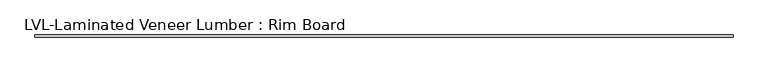
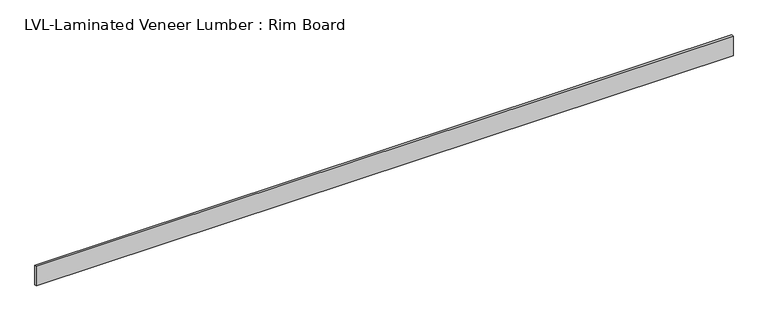
"""IFC4 building model written with IfcOpenShell, lengths in millimetres: beam geometry, LVL-Laminated Veneer Lumber : Rim Board."""

from ifc_helpers import new_model, si_unit, frame, origin, place, context, project, spatial, polyline, outline, extrude, source, transform, mapped, element, save


def lvl_laminated_veneer_lumber_rim_board_c76fbf88(model_context):
    return source(origin(), model_context, "Body", "SweptSolid", [
        extrude(outline(polyline([(5118.89375, 15.875), (5118.89375, -15.875), (-5118.89375, -15.875), (-5118.89375, 15.875), (5118.89375, 15.875)])), frame((0.0, 0.0, -150.8125), z_axis=(0.0, 0.0, 1.0), x_axis=(1.0, 0.0, 0.0)), (0.0, 0.0, 1.0), 301.625),
    ])


if __name__ == "__main__":
    model = new_model("IFC4")
    model_context = context("Model", 3, world=origin())
    ifc_project = project(units=[si_unit("LENGTHUNIT", "METRE", prefix="MILLI")], contexts=[model_context])
    site = spatial("IfcSite", under=ifc_project)
    building = spatial("IfcBuilding", under=site)
    placement = place(None, origin())
    lvl_laminated_veneer_lumber_rim_board_shape = lvl_laminated_veneer_lumber_rim_board_c76fbf88(model_context)
    element("IfcBeam", 1, ObjectType="LVL-Laminated Veneer Lumber : Rim Board", at=placement, inside=building, context=model_context, shape_type="MappedRepresentation", body=[
        mapped(lvl_laminated_veneer_lumber_rim_board_shape, transform((0.0, 0.0, 0.0), x_axis=(1.0, 0.0, 0.0), y_axis=(0.0, 1.0, 0.0), z_axis=(0.0, 0.0, 1.0))),
    ])
    save(model, "model.ifc")

# Revit data of these elements
# Type "LVL-Laminated Veneer Lumber : Rim Board"
#   Assembly Code = "B10"
#   Cost = 4.6
#   Length [instance default] = 5' - 0"
#   b = 0' - 1 1/4"
#   d = 0' - 11 7/8"
#   Structural Material [instance default] = Softwood, Lumber
# Element 1 (IfcBeam, "LVL-Laminated Veneer Lumber : Rim Board")
#   Structural Material = Douglas Fir #2
#   Materials on its faces: "Douglas Fir #2"
# Materials
#   "Softwood, Lumber": class "Wood", colour RGB 223 192 134, transparency 0, Description = "Pinus Echinata", Cost = 0
#   "Douglas Fir #2": class "Wood", colour RGB 223 192 134, transparency 0, Description = "Pinus Echinata", Cost = 0
